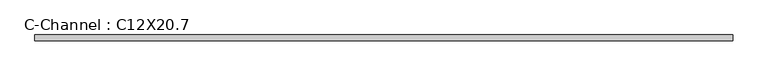
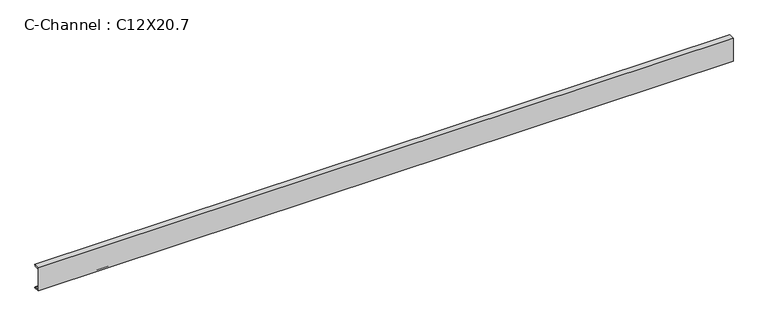
"""IFC4 building model written with IfcOpenShell, lengths in millimetres: beam geometry, C-Channel : C12X20.7."""

from ifc_helpers import new_model, si_unit, point, frame, frame_2d, origin, place, context, project, spatial, polyline, circle_curve, trimmed, segment, composite_curve, outline, extrude, source, transform, mapped, element, save


def c_channel_c12x20_7_1ea3ebde(model_context):
    return source(origin(), model_context, "Body", "SweptSolid", [
        extrude(outline(composite_curve([segment(polyline([(-17.7292, 152.4), (56.9468, 152.4)]), True, "CONTINUOUS"), segment(trimmed(circle_curve(frame_2d((44.2214, 152.4)), 12.7254), [point((56.9468, 152.4))], [point((44.2214, 139.6746))], False, "CARTESIAN"), True, "CONTINUOUS"), segment(polyline([(44.2214, 139.6746), (-10.5664, 130.997065), (-10.5664, -130.997065), (44.2214, -139.6746)]), True, "CONTINUOUS"), segment(trimmed(circle_curve(frame_2d((44.2214, -152.4)), 12.7254), [point((44.2214, -139.6746))], [point((56.9468, -152.4))], False, "CARTESIAN"), True, "CONTINUOUS"), segment(polyline([(56.9468, -152.4), (-17.7292, -152.4), (-17.7292, 152.4)]), True, "CONTINUOUS")], self_intersect=False)), frame((-4359.119673, 0.0, 0.0), z_axis=(1.0, 0.0, 0.0), x_axis=(0.0, 1.0, 0.0)), (0.0, 0.0, 1.0), 8689.063786),
    ])


if __name__ == "__main__":
    model = new_model("IFC4")
    model_context = context("Model", 3, world=origin())
    ifc_project = project(units=[si_unit("LENGTHUNIT", "METRE", prefix="MILLI")], contexts=[model_context])
    site = spatial("IfcSite", under=ifc_project)
    building = spatial("IfcBuilding", under=site)
    placement = place(None, origin())
    c_channel_c12x20_7_shape = c_channel_c12x20_7_1ea3ebde(model_context)
    element("IfcBeam", 1, ObjectType="C-Channel : C12X20.7", at=placement, inside=building, context=model_context, shape_type="MappedRepresentation", body=[
        mapped(c_channel_c12x20_7_shape, transform((0.0, 0.0, 0.0), x_axis=(1.0, 0.0, 0.0), y_axis=(0.0, 1.0, 0.0), z_axis=(0.0, 0.0, 1.0))),
    ])
    save(model, "model.ifc")

# Revit data of these elements
# Type "C-Channel : C12X20.7"
#   Assembly Code = "B10"
#   W = 20.7
#   Start Extension Calculation [instance default] = 10' - 0"
#   Start Extension [instance default] = -0' - 0 1/2"
#   End Extension Calculation [instance default] = 10' - 0"
#   End Extension [instance default] = -0' - 0 1/2"
#   Length [instance default] = 5' - 0"
#   bf = 0' - 2.94"
#   d = 1' - 0"
#   tf = 0' - 0.501"
#   tw = 0' - 0.282"
#   x = 0' - 0.698"
#   A = 0.0422222 SF
#   Structural Material [instance default] = Metal - Steel - ASTM A36
# Element 1 (IfcBeam, "C-Channel : C12X20.7")
#   Materials on its faces: "Metal - Steel - ASTM A36"
# Materials
#   "Metal - Steel - ASTM A36": class "Metal", colour RGB 199 199 199, transparency 0
